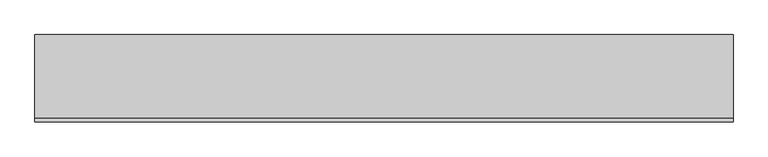
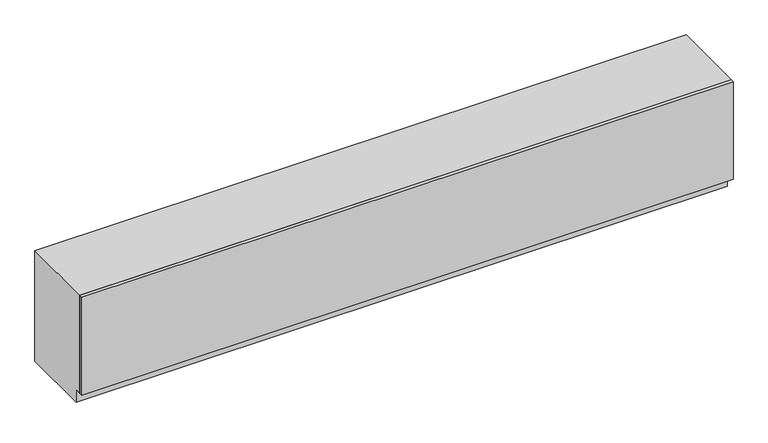
"""IFC4 building model written with IfcOpenShell, lengths in millimetres: furniture geometry, OD_CW_Base Cabinet : OD_CW_Base Cabinet."""

from ifc_helpers import new_model, si_unit, frame, origin, place, context, project, spatial, polyline, outline, extrude, source, transform, mapped, element, save


def furniture_12da59e3(model_context):
    return source(origin(), model_context, "Body", "SweptSolid", [
        extrude(outline(polyline([(18.7377049, 25.4), (4895.5377049, 25.4), (4895.5377049, 0.0), (18.7377049, 0.0), (18.7377049, 25.4)])), frame((0.0, 0.0, 101.6), z_axis=(0.0, 0.0, 1.0), x_axis=(1.0, 0.0, 0.0)), (0.0, 0.0, 1.0), 774.7),
        extrude(outline(polyline([(25.4, 876.3), (609.6, 876.3), (609.6, 0.0), (76.2, 0.0), (76.2, 101.6), (25.4, 101.6), (25.4, 876.3)])), frame((18.7377049, 0.0, 0.0), z_axis=(1.0, 0.0, 0.0), x_axis=(0.0, 1.0, 0.0)), (0.0, 0.0, 1.0), 4876.8),
    ])


if __name__ == "__main__":
    model = new_model("IFC4")
    model_context = context("Model", 3, world=origin())
    ifc_project = project(units=[si_unit("LENGTHUNIT", "METRE", prefix="MILLI")], contexts=[model_context])
    site = spatial("IfcSite", under=ifc_project)
    building = spatial("IfcBuilding", under=site)
    placement = place(None, origin())
    furniture_shape = furniture_12da59e3(model_context)
    element("IfcFurniture", 1, ObjectType="OD_CW_Base Cabinet : OD_CW_Base Cabinet", at=placement, inside=building, context=model_context, shape_type="MappedRepresentation", body=[
        mapped(furniture_shape, transform((0.0, 0.0, 0.0), x_axis=(1.0, 0.0, 0.0), y_axis=(0.0, 1.0, 0.0), z_axis=(0.0, 0.0, 1.0))),
    ])
    save(model, "model.ifc")

# Revit data of these elements
# Type "OD_CW_Base Cabinet : OD_CW_Base Cabinet"
#   OD_CW_Width [instance default] = 2' - 10"
#   OD_CW_Length [instance default] = 8' - 0"
#   OD_CW_Height [instance default] = 2' - 3"
#   Depth = 2' - 0"
#   Height = 3' - 0"
#   Width = 4' - 0"
#   OD_CW_Material_Front Panel [instance default] = none
#   OD_CW_Material_Body [instance default] = none
# Element 1 (IfcFurniture, "OD_CW_Base Cabinet : OD_CW_Base Cabinet")
#   OD_CW_Width = 2' - 0"
#   OD_CW_Length = 16' - 0"
#   OD_CW_Height = 2' - 10 1/2"
